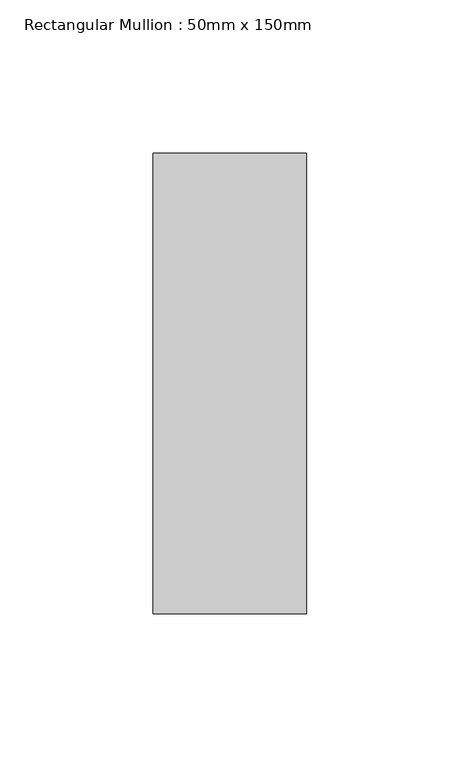
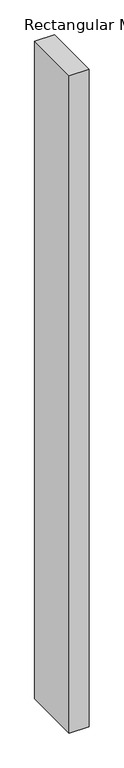
"""IFC4 building model written with IfcOpenShell, lengths in millimetres: member geometry, Rectangular Mullion : 50mm x 150mm."""

from ifc_helpers import new_model, si_unit, frame, origin, place, context, project, spatial, polyline, outline, extrude, source, transform, mapped, element, save


def rectangular_mullion_50mm_x_150mm_98166103(model_context):
    return source(origin(), model_context, "Body", "SweptSolid", [
        extrude(outline(polyline([(0.0, 75.0), (0.0, -75.0), (-50.0, -75.0), (-50.0, 75.0), (0.0, 75.0)])), frame((0.0, 0.0, -1748.5454546), z_axis=(0.0, 0.0, 1.0), x_axis=(1.0, 0.0, 0.0)), (0.0, 0.0, 1.0), 1748.5454546),
    ])


if __name__ == "__main__":
    model = new_model("IFC4")
    model_context = context("Model", 3, world=origin())
    ifc_project = project(units=[si_unit("LENGTHUNIT", "METRE", prefix="MILLI")], contexts=[model_context])
    site = spatial("IfcSite", under=ifc_project)
    building = spatial("IfcBuilding", under=site)
    placement = place(None, origin())
    rectangular_mullion_50mm_x_150mm_shape = rectangular_mullion_50mm_x_150mm_98166103(model_context)
    element("IfcMember", 1, ObjectType="Rectangular Mullion : 50mm x 150mm", at=placement, inside=building, context=model_context, shape_type="MappedRepresentation", body=[
        mapped(rectangular_mullion_50mm_x_150mm_shape, transform((0.0, 0.0, 0.0), x_axis=(1.0, 0.0, 0.0), y_axis=(0.0, 1.0, 0.0), z_axis=(0.0, 0.0, 1.0))),
    ])
    save(model, "model.ifc")

# Revit data of these elements
# Type "Rectangular Mullion : 50mm x 150mm"
#   built-in parameter 1007304 = 0.492126 (stored number, unit not read)
#   built-in parameter 1007301 = 0.082021 (stored number, unit not read)
#   built-in parameter 1007300 = 0.082021 (stored number, unit not read)
# Element 1 (IfcMember, "Rectangular Mullion : 50mm x 150mm")
#   Materials on its faces: "Aluminum"
# Materials
#   "Aluminum": class "Metal", colour RGB 244 244 244, transparency 0, Description = "Aluminum 6061", Cost = 0
